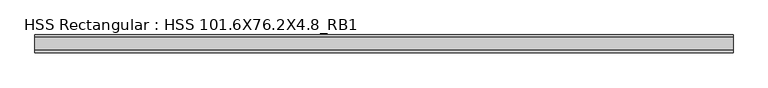
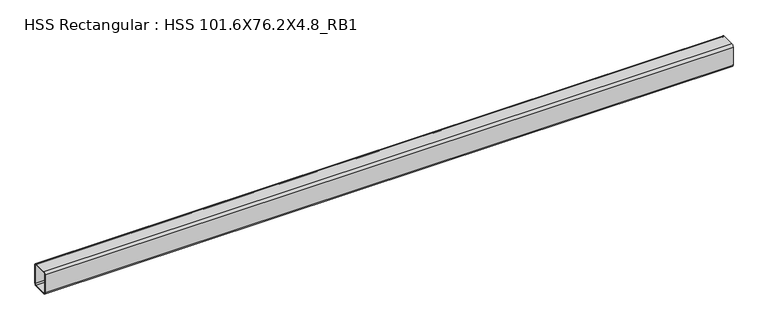
"""IFC4 building model written with IfcOpenShell, lengths in millimetres: beam geometry, HSS Rectangular : HSS 101.6X76.2X4.8_RB1."""

from ifc_helpers import new_model, si_unit, point, frame, frame_2d, origin, place, context, project, spatial, polyline, circle_curve, trimmed, segment, composite_curve, outline, extrude, source, transform, mapped, element, save


def hss_rectangular_hss_101_6x76_2x4_8_rb1_f023e725(model_context):
    return source(origin(), model_context, "Body", "SweptSolid", [
        extrude(outline(composite_curve([segment(trimmed(circle_curve(frame_2d((-28.575, 41.275)), 9.525), [point((-38.1, 41.275))], [point((-28.575, 50.8))], False, "CARTESIAN"), True, "CONTINUOUS"), segment(polyline([(-28.575, 50.8), (28.575, 50.8)]), True, "CONTINUOUS"), segment(trimmed(circle_curve(frame_2d((28.575, 41.275)), 9.525), [point((28.575, 50.8))], [point((38.1, 41.275))], False, "CARTESIAN"), True, "CONTINUOUS"), segment(polyline([(38.1, 41.275), (38.1, -41.275)]), True, "CONTINUOUS"), segment(trimmed(circle_curve(frame_2d((28.575, -41.275)), 9.525), [point((38.1, -41.275))], [point((28.575, -50.8))], False, "CARTESIAN"), True, "CONTINUOUS"), segment(polyline([(28.575, -50.8), (-28.575, -50.8)]), True, "CONTINUOUS"), segment(trimmed(circle_curve(frame_2d((-28.575, -41.275)), 9.525), [point((-28.575, -50.8))], [point((-38.1, -41.275))], False, "CARTESIAN"), True, "CONTINUOUS"), segment(polyline([(-38.1, -41.275), (-38.1, 41.275)]), True, "CONTINUOUS")], self_intersect=False), holes=[composite_curve([segment(polyline([(28.575, 46.0375), (-28.575, 46.0375)]), True, "CONTINUOUS"), segment(trimmed(circle_curve(frame_2d((-28.575, 41.275)), 4.7625), [point((-28.575, 46.0375))], [point((-33.3375, 41.275))], True, "CARTESIAN"), True, "CONTINUOUS"), segment(polyline([(-33.3375, 41.275), (-33.3375, -41.275)]), True, "CONTINUOUS"), segment(trimmed(circle_curve(frame_2d((-28.575, -41.275)), 4.7625), [point((-33.3375, -41.275))], [point((-28.575, -46.0375))], True, "CARTESIAN"), True, "CONTINUOUS"), segment(polyline([(-28.575, -46.0375), (28.575, -46.0375)]), True, "CONTINUOUS"), segment(trimmed(circle_curve(frame_2d((28.575, -41.275)), 4.7625), [point((28.575, -46.0375))], [point((33.3375, -41.275))], True, "CARTESIAN"), True, "CONTINUOUS"), segment(polyline([(33.3375, -41.275), (33.3375, 41.275)]), True, "CONTINUOUS"), segment(trimmed(circle_curve(frame_2d((28.575, 41.275)), 4.7625), [point((33.3375, 41.275))], [point((28.575, 46.0375))], True, "CARTESIAN"), True, "CONTINUOUS")], self_intersect=False)]), frame((-1525.4000006, 0.0, 0.0), z_axis=(1.0, 0.0, 0.0), x_axis=(0.0, 1.0, 0.0)), (0.0, 0.0, 1.0), 2987.3000012),
    ])


if __name__ == "__main__":
    model = new_model("IFC4")
    model_context = context("Model", 3, world=origin())
    ifc_project = project(units=[si_unit("LENGTHUNIT", "METRE", prefix="MILLI")], contexts=[model_context])
    site = spatial("IfcSite", under=ifc_project)
    building = spatial("IfcBuilding", under=site)
    placement = place(None, origin())
    hss_rectangular_hss_101_6x76_2x4_8_rb1_shape = hss_rectangular_hss_101_6x76_2x4_8_rb1_f023e725(model_context)
    element("IfcBeam", 1, ObjectType="HSS Rectangular : HSS 101.6X76.2X4.8_RB1", at=placement, inside=building, context=model_context, shape_type="MappedRepresentation", body=[
        mapped(hss_rectangular_hss_101_6x76_2x4_8_rb1_shape, transform((0.0, 0.0, 0.0), x_axis=(1.0, 0.0, 0.0), y_axis=(0.0, 1.0, 0.0), z_axis=(0.0, 0.0, 1.0))),
    ])
    save(model, "model.ifc")

# Revit data of these elements
# Type "HSS Rectangular : HSS 101.6X76.2X4.8_RB1"
#   Section Name Key = "HSS 4X3X3/16"
#   Assembly Code = "B10"
#   Width = 7.62 cm
#   Wall Nominal Thickness = 0.4763 cm
#   Wall Design Thickness = 0.442 cm
#   Torsional Moment of Inertia = 260.561 cm⁴
#   Torsional Modulus = 61.2876 cm³
#   Section Area = 14.4516 cm²
#   Plastic Modulus weak axis = 40.3122 cm³
#   Plastic Modulus strong axis = 49.1612 cm³
#   Perimeter = 0.881482 m²/m
#   Outer Fillet = 0.9525 cm
#   Nominal Weight = 12.1285 kgf/m
#   Moment of Inertia weak axis = 131.529 cm⁴
#   Moment of Inertia strong axis = 205.202 cm⁴
#   Inner Fillet = 0.4763 cm
#   Height = 10.16 cm
#   Elastic Modulus weak axis = 34.4128 cm³
#   Elastic Modulus strong axis = 40.476 cm³
#   Centroid Vertical = 5.08 cm
#   Centroid Horizontal = 3.81 cm
#   Length [instance default] = 1524 mm
#   Structural Material [instance default] = Steel ASTM A500, Grade B, Rectangular and Square
#   Principal Axes Angle = 0
# Element 1 (IfcBeam, "HSS Rectangular : HSS 101.6X76.2X4.8_RB1")
#   Structural Material = Steel ASTM A992
#   Materials on its faces: "Steel ASTM A992"
# Materials
#   "Steel ASTM A500, Grade B, Rectangular and Square": class "Metal", colour RGB 199 199 199, transparency 0, Description = "Carbon steel", Cost = 0
#   "Steel ASTM A992": class "Metal", colour RGB 199 199 199, transparency 0, Description = "Structural steel 50ksi", Cost = 0
